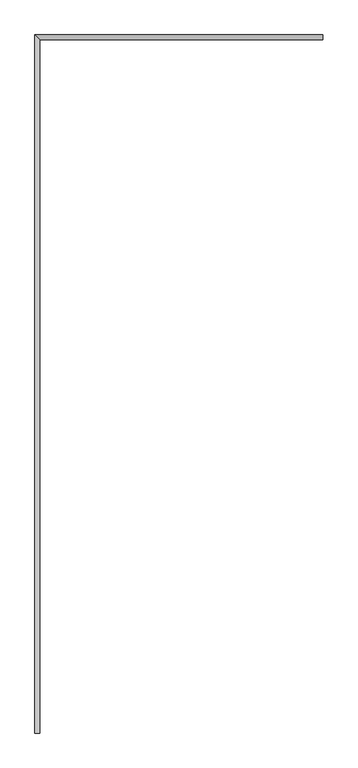
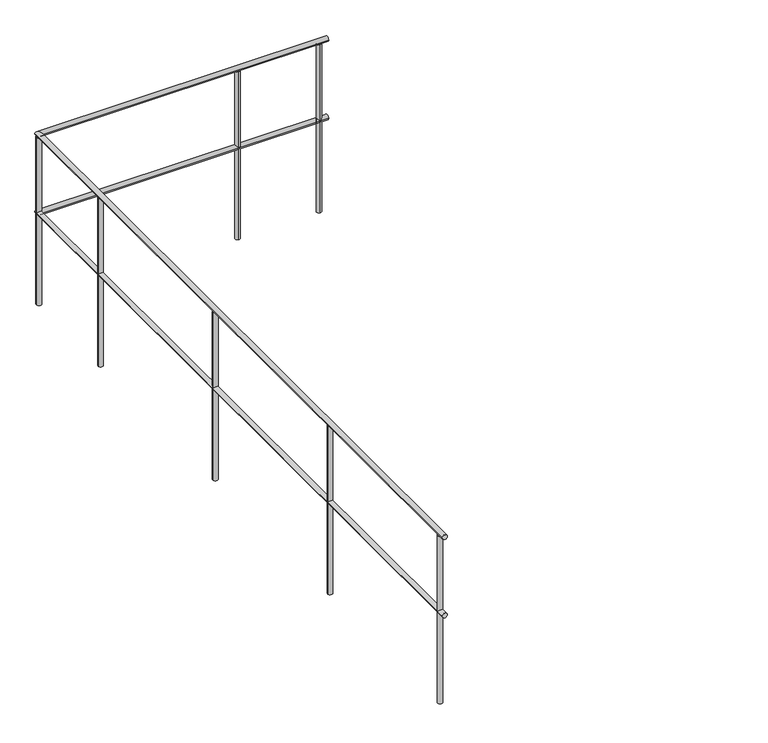
"""IFC4 building model written with IfcOpenShell, lengths in millimetres: railing geometry."""

import ifcopenshell
import ifcopenshell.guid

model = None  # the IFC model being written
_history = None  # IfcOwnerHistory: only IFC2X3 demands one
_inside = {}  # id of a spatial element -> (the spatial element, [elements in it])
_under = {}  # id of a project, library or spatial element -> (it, [spatial elements below it])
_declared = {}  # id of a project -> (the project, [libraries it declares])
_typed = {}  # id of a type object -> (the type object, [elements of that type])
_made_of = {}  # id of a material, layer set ... -> (it, [elements and type objects made of it])


def new_model(schema):
    """Start an empty IFC model of exactly this schema.

    Asked for "IFC4X3", IfcOpenShell would pick the latest addendum, in which some entities
    have other attributes; the version numbers below select the first issue.
    IFC2X3 requires an IfcOwnerHistory on every rooted entity: one is made here for all.
    """
    global model, _history
    if schema == "IFC4X3":
        model = ifcopenshell.file(schema_version=(4, 3, 0, 0))
    else:
        model = ifcopenshell.file(schema=schema)
    _inside.clear()
    _under.clear()
    _declared.clear()
    _typed.clear()
    _made_of.clear()
    _history = None
    if model.schema == "IFC2X3":
        org = make("IfcOrganization", Name="unknown")
        user = make(
            "IfcPersonAndOrganization",
            ThePerson=make("IfcPerson", FamilyName="unknown"),
            TheOrganization=org,
        )
        app = make(
            "IfcApplication",
            ApplicationDeveloper=org,
            Version="unknown",
            ApplicationFullName="unknown",
            ApplicationIdentifier="unknown",
        )
        _history = make(
            "IfcOwnerHistory",
            OwningUser=user,
            OwningApplication=app,
            ChangeAction="ADDED",
            CreationDate=0,
        )
    return model


def make(cls, **values):
    """One entity of the class cls with the attributes given. An attribute that is None is left unset."""
    return model.create_entity(
        cls, **{name: value for name, value in values.items() if value is not None}
    )


def rooted(cls, **values):
    """An entity with a GlobalId (a new one), such as an element, a storey or a relation."""
    return make(cls, GlobalId=ifcopenshell.guid.new(), OwnerHistory=_history, **values)


def si_unit(unit_type, name, prefix=None):
    """IfcSIUnit, for example si_unit("LENGTHUNIT", "METRE", prefix="MILLI")."""
    return make("IfcSIUnit", UnitType=unit_type, Prefix=prefix, Name=name)


def assignment(units):
    """IfcUnitAssignment: the units of a project."""
    return None if units is None else make("IfcUnitAssignment", Units=units)


def point(xyz):
    """IfcCartesianPoint."""
    return None if xyz is None else make("IfcCartesianPoint", Coordinates=xyz)


def direction(xyz):
    """IfcDirection."""
    return None if xyz is None else make("IfcDirection", DirectionRatios=xyz)


def frame(location, z_axis=None, x_axis=None):
    """IfcAxis2Placement3D, a coordinate frame: its origin and axes. An axis left out is left unset."""
    return make(
        "IfcAxis2Placement3D",
        Location=point(location),
        Axis=direction(z_axis),
        RefDirection=direction(x_axis),
    )


def frame_2d(location, x_axis=None):
    """IfcAxis2Placement2D, a coordinate frame in the plane: its origin and x axis."""
    return make(
        "IfcAxis2Placement2D", Location=point(location), RefDirection=direction(x_axis)
    )


def origin():
    """The frame at (0, 0, 0) with its axes left unset."""
    return frame((0.0, 0.0, 0.0))


def place(relative_to, where):
    """IfcLocalPlacement: puts the frame where relative to a parent placement (None: the world)."""
    return make(
        "IfcLocalPlacement", PlacementRelTo=relative_to, RelativePlacement=where
    )


def context(
    kind, dimensions, precision=None, world=None, true_north=None, identifier=None
):
    """IfcGeometricRepresentationContext, for example the 3D "Model" context."""
    return make(
        "IfcGeometricRepresentationContext",
        ContextIdentifier=identifier,
        ContextType=kind,
        CoordinateSpaceDimension=dimensions,
        Precision=precision,
        WorldCoordinateSystem=world,
        TrueNorth=true_north,
    )


def project(units=None, contexts=None):
    """IfcProject with its units and contexts."""
    return rooted(
        "IfcProject",
        Name="project",
        RepresentationContexts=contexts,
        UnitsInContext=assignment(units),
    )


def spatial(cls, under=None, at=None, **own):
    """A site, building, storey or space (cls), placed at a placement, below another one or the project."""
    s = rooted(cls, ObjectPlacement=at, **own)
    if under is not None:
        _under.setdefault(under.id(), (under, []))[1].append(s)
    return s


def circle_curve(where, radius):
    """IfcCircle in the frame where."""
    return make("IfcCircle", Position=where, Radius=radius)


def ellipse_curve(where, semi_axis1, semi_axis2):
    """IfcEllipse in the frame where."""
    return make(
        "IfcEllipse", Position=where, SemiAxis1=semi_axis1, SemiAxis2=semi_axis2
    )


def trimmed(basis, trim1, trim2, sense, master):
    """IfcTrimmedCurve: the piece of a basis curve between two trims."""
    return make(
        "IfcTrimmedCurve",
        BasisCurve=basis,
        Trim1=trim1,
        Trim2=trim2,
        SenseAgreement=sense,
        MasterRepresentation=master,
    )


def segment(curve, same_sense, transition):
    """IfcCompositeCurveSegment."""
    return make(
        "IfcCompositeCurveSegment",
        Transition=transition,
        SameSense=same_sense,
        ParentCurve=curve,
    )


def composite_curve(segments, self_intersect=None):
    """IfcCompositeCurve: segments joined end to end."""
    return make("IfcCompositeCurve", Segments=segments, SelfIntersect=self_intersect)


def outline(outer, holes=None, kind="AREA"):
    """IfcArbitraryClosedProfileDef: a profile drawn as a closed curve; with holes, ...WithVoids."""
    if holes is None:
        return make("IfcArbitraryClosedProfileDef", ProfileType=kind, OuterCurve=outer)
    return make(
        "IfcArbitraryProfileDefWithVoids",
        ProfileType=kind,
        OuterCurve=outer,
        InnerCurves=holes,
    )


def extrude(swept, where, along, depth):
    """IfcExtrudedAreaSolid: the profile swept, set in the frame where, extruded along a direction by depth."""
    return make(
        "IfcExtrudedAreaSolid",
        SweptArea=swept,
        Position=where,
        ExtrudedDirection=direction(along),
        Depth=depth,
    )


def shape(context_of_items, identifier, shape_type, items):
    """IfcShapeRepresentation: the items that make up one representation, for example the "Body"."""
    return make(
        "IfcShapeRepresentation",
        ContextOfItems=context_of_items,
        RepresentationIdentifier=identifier,
        RepresentationType=shape_type,
        Items=items,
    )


def source(mapping_origin, context_of_items, identifier, shape_type, items):
    """IfcRepresentationMap: a shape defined once, which mapped items show again and again."""
    return make(
        "IfcRepresentationMap",
        MappingOrigin=mapping_origin,
        MappedRepresentation=shape(context_of_items, identifier, shape_type, items),
    )


def transform(
    local_origin,
    x_axis=None,
    y_axis=None,
    z_axis=None,
    scale=None,
    scale2=None,
    scale3=None,
    uniform=True,
):
    """IfcCartesianTransformationOperator3D, or its non-uniform kind. x_axis, y_axis, z_axis: its Axis1, 2, 3."""
    if uniform:
        return make(
            "IfcCartesianTransformationOperator3D",
            Axis1=direction(x_axis),
            Axis2=direction(y_axis),
            LocalOrigin=point(local_origin),
            Scale=scale,
            Axis3=direction(z_axis),
        )
    return make(
        "IfcCartesianTransformationOperator3DnonUniform",
        Axis1=direction(x_axis),
        Axis2=direction(y_axis),
        LocalOrigin=point(local_origin),
        Scale=scale,
        Axis3=direction(z_axis),
        Scale2=scale2,
        Scale3=scale3,
    )


def mapped(mapping_source, mapping_target):
    """IfcMappedItem: shows the shape of a source again, moved by a transform."""
    return make(
        "IfcMappedItem", MappingSource=mapping_source, MappingTarget=mapping_target
    )


def made_of(thing, what):
    """Note that an element or type object is made of a material, layer set ...; save() writes the relation."""
    if what is not None:
        _made_of.setdefault(what.id(), (what, []))[1].append(thing)
    return thing


def element(
    cls,
    number,
    at=None,
    inside=None,
    cuts=None,
    type_object=None,
    material=None,
    context=None,
    identifier="Body",
    shape_type=None,
    held_by="IfcProductDefinitionShape",
    body=None,
    shapes=None,
    **own,
):
    """One element of the class cls, such as IfcWall. Its Tag is "e" and its number.

    at: its placement. inside: the storey or other place that contains it. cuts: it is an
    opening in that element (IfcRelVoidsElement). A single representation is given by context,
    identifier, shape_type and body (its items); several are given by shapes. held_by: the class
    of the entity that holds the representations. save() writes the other relations.
    """
    e = rooted(cls, Tag="e%d" % number, ObjectPlacement=at, **own)
    if body is not None:
        shapes = [shape(context, identifier, shape_type, body)]
    if shapes is not None:
        e.Representation = make(held_by, Representations=shapes)
    if inside is not None:
        _inside.setdefault(inside.id(), (inside, []))[1].append(e)
    if cuts is not None:
        rooted(
            "IfcRelVoidsElement", RelatingBuildingElement=cuts, RelatedOpeningElement=e
        )
    if type_object is not None:
        _typed.setdefault(type_object.id(), (type_object, []))[1].append(e)
    return made_of(e, material)


def aggregate(whole, parts):
    """IfcRelAggregates: a whole, such as a stair, and the parts it consists of."""
    return rooted("IfcRelAggregates", RelatingObject=whole, RelatedObjects=parts)


def save(model, path):
    """Write the relations noted so far, then the file.

    IfcRelAggregates (storeys below a building ...), IfcRelContainedInSpatialStructure (elements
    in a storey), IfcRelDefinesByType, IfcRelAssociatesMaterial and IfcRelDeclares: one each for
    every whole, place, type object, material and project.
    """
    for whole, parts in _under.values():
        aggregate(whole, parts)
    for where, things in _inside.values():
        rooted(
            "IfcRelContainedInSpatialStructure",
            RelatedElements=things,
            RelatingStructure=where,
        )
    for kind, things in _typed.values():
        rooted("IfcRelDefinesByType", RelatedObjects=things, RelatingType=kind)
    for what, things in _made_of.values():
        rooted("IfcRelAssociatesMaterial", RelatedObjects=things, RelatingMaterial=what)
    for by, libraries in _declared.values():
        rooted("IfcRelDeclares", RelatingContext=by, RelatedDefinitions=libraries)
    model.write(path)


def plane_surface(at):
    """IfcPlane: the flat surface through the origin of the frame at, square to its z axis."""
    return make("IfcPlane", Position=at)


def cylinder_surface(at, radius):
    """IfcCylindricalSurface: all points at the distance radius from the z axis of the frame at."""
    return make("IfcCylindricalSurface", Position=at, Radius=radius)


def advanced_brep(points, edges, surfaces, faces):
    """IfcAdvancedBrep: a solid bounded by faces that lie on surfaces and meet in shared edges.

    An edge is (start, end): straight between two places in points (the first is 0);
    or (start, end, curve); or (start, end, curve, False) where it runs against its curve.
    A face is (place in surfaces, loops), or (place, loops, False) where it looks against
    its surface's normal. A loop lists edges by number (the first is 1), with a minus sign
    where the edge is run from its end to its start. The first loop is the outer one.
    """
    corners = [point(p) for p in points]
    vertices = [make("IfcVertexPoint", VertexGeometry=c) for c in corners]
    made = []
    for start, end, *more in edges:
        made.append(
            make(
                "IfcEdgeCurve",
                EdgeStart=vertices[start],
                EdgeEnd=vertices[end],
                EdgeGeometry=more[0] if more else make("IfcPolyline", Points=[corners[start], corners[end]]),
                SameSense=more[1] if len(more) > 1 else True,
            )
        )
    hull = []
    for where, loops, *sense in faces:
        bounds = []
        for j, loop in enumerate(loops):
            ring = [make("IfcOrientedEdge", EdgeElement=made[abs(k) - 1], Orientation=k > 0) for k in loop]
            bounds.append(
                make(
                    "IfcFaceOuterBound" if j == 0 else "IfcFaceBound",
                    Bound=make("IfcEdgeLoop", EdgeList=ring),
                    Orientation=True,
                )
            )
        hull.append(make("IfcAdvancedFace", Bounds=bounds, FaceSurface=surfaces[where], SameSense=sense[0] if sense else True))
    return make("IfcAdvancedBrep", Outer=make("IfcClosedShell", CfsFaces=hull))


def railing_0adeda9c(model_context):
    return source(origin(), model_context, "Body", "SolidModel", [
        advanced_brep(
        [(-2206.0, 48114.2482382, 885.0), (-2176.0, 48114.2482382, 885.0), (-2206.0, 52374.7934796, 885.0), (-2176.0, 52344.7934796, 885.0), (-450.0, 52374.7934796, 885.0), (-450.0, 52344.7934796, 885.0)],
        [
            (0, 1, circle_curve(frame((-2191.0, 48114.2482382, 885.0), z_axis=(0.0, -1.0, 0.0), x_axis=(1.0, 0.0, 0.0)), 15.0)),
            (1, 0, circle_curve(frame((-2191.0, 48114.2482382, 885.0), z_axis=(0.0, -1.0, 0.0), x_axis=(1.0, 0.0, 0.0)), 15.0)),
            (0, 2),
            (2, 3, ellipse_curve(frame((-2191.0, 52359.7934796, 885.0), z_axis=(-0.7071067811865498, -0.7071067811865452, 0.0), x_axis=(0.7071067811865452, -0.7071067811865499, 0.0)), 21.2132034, 15.0)),
            (3, 1),
            (3, 2, ellipse_curve(frame((-2191.0, 52359.7934796, 885.0), z_axis=(-0.7071067811865498, -0.7071067811865452, 0.0), x_axis=(0.7071067811865452, -0.7071067811865499, 0.0)), 21.2132034, 15.0)),
            (4, 5, circle_curve(frame((-450.0, 52359.7934796, 885.0), z_axis=(1.0, 0.0, 0.0), x_axis=(0.0, -1.0, 0.0)), 15.0)),
            (5, 4, circle_curve(frame((-450.0, 52359.7934796, 885.0), z_axis=(1.0, 0.0, 0.0), x_axis=(0.0, -1.0, 0.0)), 15.0)),
            (2, 4),
            (5, 3),
        ],
        [
            plane_surface(frame((-2191.0, 48114.2482382, 900.0), z_axis=(0.0, -1.0, 0.0), x_axis=(0.0, 0.0, 1.0))),
            cylinder_surface(frame((-2191.0, 48114.2482382, 885.0), z_axis=(0.0, -1.0, 0.0), x_axis=(1.0, 0.0, 0.0)), 15.0),
            plane_surface(frame((-450.0, 52359.7934796, 900.0), z_axis=(1.0, 0.0, 0.0), x_axis=(0.0, 1.0, 0.0))),
            cylinder_surface(frame((-2191.0, 52359.7934796, 885.0), z_axis=(-1.0, 0.0, 0.0), x_axis=(0.0, -1.0, 0.0)), 15.0),
        ],
        [
            (0, [[1, 2]]),
            (1, [[-1, 3, 4, 5]]),
            (1, [[-2, -5, 6, -3]]),
            (2, [[7, 8]]),
            (3, [[-4, 9, -8, 10]]),
            (3, [[-6, -10, -7, -9]]),
        ],
    ),
        advanced_brep(
        [(-2206.0, 48114.2482382, 1385.0), (-2176.0, 48114.2482382, 1385.0), (-2206.0, 52374.7934796, 1385.0), (-2176.0, 52344.7934796, 1385.0), (-450.0, 52374.7934796, 1385.0), (-450.0, 52344.7934796, 1385.0)],
        [
            (0, 1, circle_curve(frame((-2191.0, 48114.2482382, 1385.0), z_axis=(0.0, -1.0, 0.0), x_axis=(1.0, 0.0, 0.0)), 15.0)),
            (1, 0, circle_curve(frame((-2191.0, 48114.2482382, 1385.0), z_axis=(0.0, -1.0, 0.0), x_axis=(1.0, 0.0, 0.0)), 15.0)),
            (0, 2),
            (2, 3, ellipse_curve(frame((-2191.0, 52359.7934796, 1385.0), z_axis=(-0.7071067811865498, -0.7071067811865452, 0.0), x_axis=(0.7071067811865452, -0.7071067811865499, 0.0)), 21.2132034, 15.0)),
            (3, 1),
            (3, 2, ellipse_curve(frame((-2191.0, 52359.7934796, 1385.0), z_axis=(-0.7071067811865498, -0.7071067811865452, 0.0), x_axis=(0.7071067811865452, -0.7071067811865499, 0.0)), 21.2132034, 15.0)),
            (4, 5, circle_curve(frame((-450.0, 52359.7934796, 1385.0), z_axis=(1.0, 0.0, 0.0), x_axis=(0.0, -1.0, 0.0)), 15.0)),
            (5, 4, circle_curve(frame((-450.0, 52359.7934796, 1385.0), z_axis=(1.0, 0.0, 0.0), x_axis=(0.0, -1.0, 0.0)), 15.0)),
            (2, 4),
            (5, 3),
        ],
        [
            plane_surface(frame((-2191.0, 48114.2482382, 1400.0), z_axis=(0.0, -1.0, 0.0), x_axis=(0.0, 0.0, 1.0))),
            cylinder_surface(frame((-2191.0, 48114.2482382, 1385.0), z_axis=(0.0, -1.0, 0.0), x_axis=(1.0, 0.0, 0.0)), 15.0),
            plane_surface(frame((-450.0, 52359.7934796, 1400.0), z_axis=(1.0, 0.0, 0.0), x_axis=(0.0, 1.0, 0.0))),
            cylinder_surface(frame((-2191.0, 52359.7934796, 1385.0), z_axis=(-1.0, 0.0, 0.0), x_axis=(0.0, -1.0, 0.0)), 15.0),
        ],
        [
            (0, [[1, 2]]),
            (1, [[-1, 3, 4, 5]]),
            (1, [[-2, -5, 6, -3]]),
            (2, [[7, 8]]),
            (3, [[-4, 9, -8, 10]]),
            (3, [[-6, -10, -7, -9]]),
        ],
    ),
        extrude(outline(composite_curve([segment(trimmed(circle_curve(frame_2d((-991.0, 52359.7934796)), 15.0), [point((-991.0, 52374.7934796))], [point((-991.0, 52344.7934796))], False, "CARTESIAN"), True, "CONTINUOUS"), segment(trimmed(circle_curve(frame_2d((-991.0, 52359.7934796)), 15.0), [point((-991.0, 52344.7934796))], [point((-991.0, 52374.7934796))], False, "CARTESIAN"), True, "CONTINUOUS")], self_intersect=False)), frame((0.0, 0.0, 300.0), z_axis=(0.0, 0.0, 1.0), x_axis=(1.0, 0.0, 0.0)), (0.0, 0.0, 1.0), 1070.0),
        extrude(outline(composite_curve([segment(trimmed(circle_curve(frame_2d((-2191.0, 51714.2482382)), 15.0), [point((-2206.0, 51714.2482382))], [point((-2176.0, 51714.2482382))], False, "CARTESIAN"), True, "CONTINUOUS"), segment(trimmed(circle_curve(frame_2d((-2191.0, 51714.2482382)), 15.0), [point((-2176.0, 51714.2482382))], [point((-2206.0, 51714.2482382))], False, "CARTESIAN"), True, "CONTINUOUS")], self_intersect=False)), frame((0.0, 0.0, 300.0), z_axis=(0.0, 0.0, 1.0), x_axis=(1.0, 0.0, 0.0)), (0.0, 0.0, 1.0), 1070.0),
        extrude(outline(composite_curve([segment(trimmed(circle_curve(frame_2d((-2191.0, 50514.2482382)), 15.0), [point((-2206.0, 50514.2482382))], [point((-2176.0, 50514.2482382))], False, "CARTESIAN"), True, "CONTINUOUS"), segment(trimmed(circle_curve(frame_2d((-2191.0, 50514.2482382)), 15.0), [point((-2176.0, 50514.2482382))], [point((-2206.0, 50514.2482382))], False, "CARTESIAN"), True, "CONTINUOUS")], self_intersect=False)), frame((0.0, 0.0, 300.0), z_axis=(0.0, 0.0, 1.0), x_axis=(1.0, 0.0, 0.0)), (0.0, 0.0, 1.0), 1070.0),
        extrude(outline(composite_curve([segment(trimmed(circle_curve(frame_2d((-2191.0, 49314.2482382)), 15.0), [point((-2206.0, 49314.2482382))], [point((-2176.0, 49314.2482382))], False, "CARTESIAN"), True, "CONTINUOUS"), segment(trimmed(circle_curve(frame_2d((-2191.0, 49314.2482382)), 15.0), [point((-2176.0, 49314.2482382))], [point((-2206.0, 49314.2482382))], False, "CARTESIAN"), True, "CONTINUOUS")], self_intersect=False)), frame((0.0, 0.0, 300.0), z_axis=(0.0, 0.0, 1.0), x_axis=(1.0, 0.0, 0.0)), (0.0, 0.0, 1.0), 1070.0),
        extrude(outline(composite_curve([segment(trimmed(circle_curve(frame_2d((-2191.0, 52359.7934796)), 15.0), [point((-2206.0, 52359.7934796))], [point((-2176.0, 52359.7934796))], False, "CARTESIAN"), True, "CONTINUOUS"), segment(trimmed(circle_curve(frame_2d((-2191.0, 52359.7934796)), 15.0), [point((-2176.0, 52359.7934796))], [point((-2206.0, 52359.7934796))], False, "CARTESIAN"), True, "CONTINUOUS")], self_intersect=False)), frame((0.0, 0.0, 300.0), z_axis=(0.0, 0.0, 1.0), x_axis=(1.0, 0.0, 0.0)), (0.0, 0.0, 1.0), 1070.0),
        extrude(outline(composite_curve([segment(trimmed(circle_curve(frame_2d((-500.0, 52359.7934796)), 15.0), [point((-500.0, 52374.7934796))], [point((-500.0, 52344.7934796))], False, "CARTESIAN"), True, "CONTINUOUS"), segment(trimmed(circle_curve(frame_2d((-500.0, 52359.7934796)), 15.0), [point((-500.0, 52344.7934796))], [point((-500.0, 52374.7934796))], False, "CARTESIAN"), True, "CONTINUOUS")], self_intersect=False)), frame((0.0, 0.0, 300.0), z_axis=(0.0, 0.0, 1.0), x_axis=(1.0, 0.0, 0.0)), (0.0, 0.0, 1.0), 1070.0),
        extrude(outline(composite_curve([segment(trimmed(circle_curve(frame_2d((-2191.0, 48164.2482382)), 15.0), [point((-2206.0, 48164.2482382))], [point((-2176.0, 48164.2482382))], False, "CARTESIAN"), True, "CONTINUOUS"), segment(trimmed(circle_curve(frame_2d((-2191.0, 48164.2482382)), 15.0), [point((-2176.0, 48164.2482382))], [point((-2206.0, 48164.2482382))], False, "CARTESIAN"), True, "CONTINUOUS")], self_intersect=False)), frame((0.0, 0.0, 300.0), z_axis=(0.0, 0.0, 1.0), x_axis=(1.0, 0.0, 0.0)), (0.0, 0.0, 1.0), 1070.0),
    ])


if __name__ == "__main__":
    model = new_model("IFC4")
    model_context = context("Model", 3, world=origin())
    ifc_project = project(units=[si_unit("LENGTHUNIT", "METRE", prefix="MILLI")], contexts=[model_context])
    site = spatial("IfcSite", under=ifc_project)
    building = spatial("IfcBuilding", under=site)
    placement = place(None, origin())
    railing_shape = railing_0adeda9c(model_context)
    element("IfcRailing", 1, at=placement, inside=building, context=model_context, shape_type="MappedRepresentation", body=[
        mapped(railing_shape, transform((0.0, 0.0, 0.0), x_axis=(1.0, 0.0, 0.0), y_axis=(0.0, 1.0, 0.0), z_axis=(0.0, 0.0, 1.0))),
    ])
    save(model, "model.ifc")
